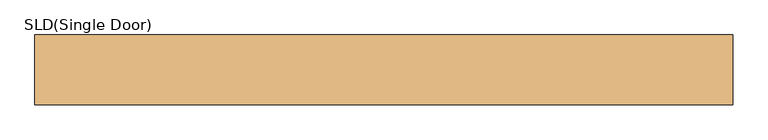
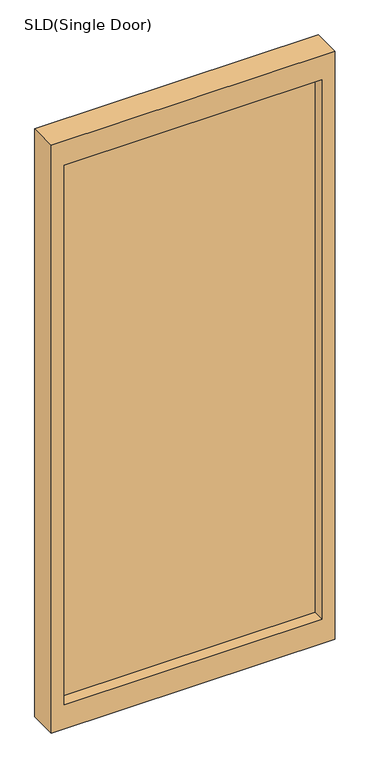
"""IFC4 building model written with IfcOpenShell, lengths in millimetres: door geometry, SLD(Single Door) : H_DR_AR B12_Door_Single_Glass_W980xH2200_SLD-1."""

from ifc_helpers import new_model, si_unit, frame, origin, place, context, project, spatial, polyline, outline, extrude, source, transform, mapped, element, save


def sld_single_door_5abaadf5(model_context):
    return source(origin(), model_context, "Body", "SweptSolid", [
        extrude(outline(polyline([(-55.0, -108.0), (-965.0, -108.0), (-965.0, -92.0), (-55.0, -92.0), (-55.0, -108.0)])), frame((0.0, 0.0, 90.0), z_axis=(0.0, 0.0, 1.0), x_axis=(1.0, 0.0, 0.0)), (0.0, 0.0, 1.0), 2010.0),
        extrude(outline(polyline([(2190.0, -10.0), (2190.0, -1010.0), (0.0, -1010.0), (0.0, -10.0), (2190.0, -10.0)]), holes=[polyline([(2100.0, -55.0), (90.0, -55.0), (90.0, -965.0), (2100.0, -965.0), (2100.0, -55.0)])]), frame((0.0, -150.0, 0.0), z_axis=(0.0, 1.0, 0.0), x_axis=(0.0, 0.0, 1.0)), (0.0, 0.0, 1.0), 100.0),
    ])


if __name__ == "__main__":
    model = new_model("IFC4")
    model_context = context("Model", 3, world=origin())
    ifc_project = project(units=[si_unit("LENGTHUNIT", "METRE", prefix="MILLI")], contexts=[model_context])
    site = spatial("IfcSite", under=ifc_project)
    building = spatial("IfcBuilding", under=site)
    placement = place(None, origin())
    sld_single_door_shape = sld_single_door_5abaadf5(model_context)
    element("IfcDoor", 1, ObjectType="SLD(Single Door) : H_DR_AR B12_Door_Single_Glass_W980xH2200_SLD-1", at=placement, inside=building, context=model_context, shape_type="MappedRepresentation", body=[
        mapped(sld_single_door_shape, transform((0.0, 0.0, 0.0), x_axis=(1.0, 0.0, 0.0), y_axis=(0.0, 1.0, 0.0), z_axis=(0.0, 0.0, 1.0))),
    ])
    save(model, "model.ifc")

# Revit data of these elements
# Type "SLD(Single Door) : H_DR_AR B12_Door_Single_Glass_W980xH2200_SLD-1"
#   Type Mark = "456"
#   Type Comments = "PD"
#   Analytic Construction = "<None>"
#   Thickness = 45 mm
#   Frame Projection Ext. = 25 mm
#   Frame Projection Int. = 25 mm
#   Frame Width = 75 mm
#   Height = 2200 mm
#   Width = 1020 mm
#   Door Width = 1000 mm
#   Door Frame Thk = 100 mm
#   Center [instance default] = 93 mm
#   Define Thermal Properties by = 1
#   Function = (empty or 0)
#   Wall Closure = (empty or 0)
# Element 1 (IfcDoor, "SLD(Single Door) : H_DR_AR B12_Door_Single_Glass_W980xH2200_SLD-1")
#   Center = 50 mm
#   Materials on its faces: "00_Metal_Stainless Steel", "00_Glass_Glass"
# Materials
#   "00_Metal_Stainless Steel": class "Metal", colour RGB 148 148 148, transparency 0, Description = "Steel", Cost = 0
#   "00_Glass_Glass": class "Glass", colour RGB 218 227 224, transparency 0.85, Description = "Glass", Cost = 0, Image = none
